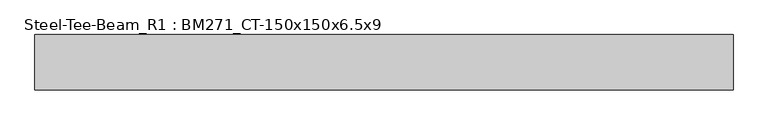
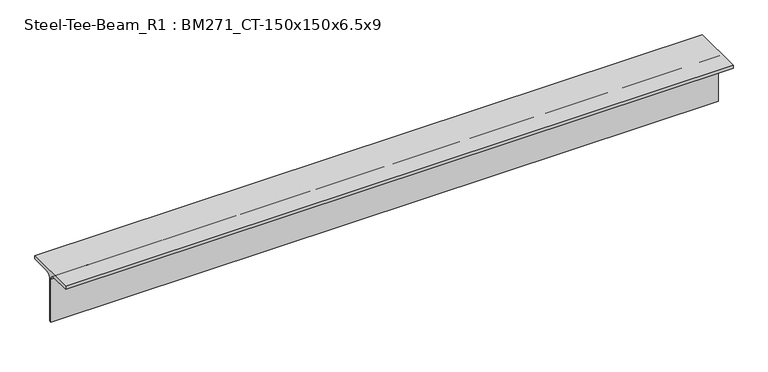
"""IFC4 building model written with IfcOpenShell, lengths in millimetres: member geometry, Steel-Tee-Beam_R1 : BM271_CT-150x150x6.5x9."""

from ifc_helpers import new_model, si_unit, point, frame, frame_2d, origin, place, context, project, spatial, polyline, circle_curve, trimmed, segment, composite_curve, outline, extrude, source, transform, mapped, element, save


def steel_tee_beam_r1_bm271_ct_150x150x6_5x9_a8473fa1(model_context):
    return source(origin(), model_context, "Body", "SweptSolid", [
        extrude(outline(composite_curve([segment(polyline([(-75.0, 75.0), (75.0, 75.0), (75.0, 66.0), (16.25, 66.0)]), True, "CONTINUOUS"), segment(trimmed(circle_curve(frame_2d((16.25, 53.0)), 13.0), [point((16.25, 66.0))], [point((3.25, 53.0))], True, "CARTESIAN"), True, "CONTINUOUS"), segment(polyline([(3.25, 53.0), (3.25, -75.0), (-3.25, -75.0), (-3.25, 53.0)]), True, "CONTINUOUS"), segment(trimmed(circle_curve(frame_2d((-16.25, 53.0)), 13.0), [point((-3.25, 53.0))], [point((-16.25, 66.0))], True, "CARTESIAN"), True, "CONTINUOUS"), segment(polyline([(-16.25, 66.0), (-75.0, 66.0), (-75.0, 75.0)]), True, "CONTINUOUS")], self_intersect=False)), frame((-900.1288904, 0.0, 0.0), z_axis=(1.0, 0.0, 0.0), x_axis=(0.0, 1.0, 0.0)), (0.0, 0.0, 1.0), 1884.11033),
    ])


if __name__ == "__main__":
    model = new_model("IFC4")
    model_context = context("Model", 3, world=origin())
    ifc_project = project(units=[si_unit("LENGTHUNIT", "METRE", prefix="MILLI")], contexts=[model_context])
    site = spatial("IfcSite", under=ifc_project)
    building = spatial("IfcBuilding", under=site)
    placement = place(None, origin())
    steel_tee_beam_r1_bm271_ct_150x150x6_5x9_shape = steel_tee_beam_r1_bm271_ct_150x150x6_5x9_a8473fa1(model_context)
    element("IfcMember", 1, ObjectType="Steel-Tee-Beam_R1 : BM271_CT-150x150x6.5x9", at=placement, inside=building, context=model_context, shape_type="MappedRepresentation", body=[
        mapped(steel_tee_beam_r1_bm271_ct_150x150x6_5x9_shape, transform((0.0, 0.0, 0.0), x_axis=(1.0, 0.0, 0.0), y_axis=(0.0, 1.0, 0.0), z_axis=(0.0, 0.0, 1.0))),
    ])
    save(model, "model.ifc")

# Revit data of these elements
# Type "Steel-Tee-Beam_R1 : BM271_CT-150x150x6.5x9"
#   Keynote = "CT-150x150x6.5x9"
#   Surface Area = 0.588841 m²/m
#   Section Area = 23.3904 cm²
#   Mass per Unit Length = 18.3614 kg/m
#   Length [instance default] = 1.5240 m
#   bf = 0.1500 m
#   d = 0.1500 m
#   k = 0.0220 m
#   r = 0.0130 m
#   tf = 0.0090 m
#   tw = 0.0065 m
#   hec_material4 [instance default] = none
#   hec_material3 [instance default] = none
#   hec_material2 [instance default] = none
#   hec_material1 [instance default] = none
#   Structural Material [instance default] = Steel, 45-345
#   Assembly Code = ""
# Element 1 (IfcMember, "Steel-Tee-Beam_R1 : BM271_CT-150x150x6.5x9")
#   Structural Material = none
# Materials
#   "Steel, 45-345": class "Metal", colour RGB 189 187 185, transparency 0, Description = "Steel 345 MPa", Cost = 0
